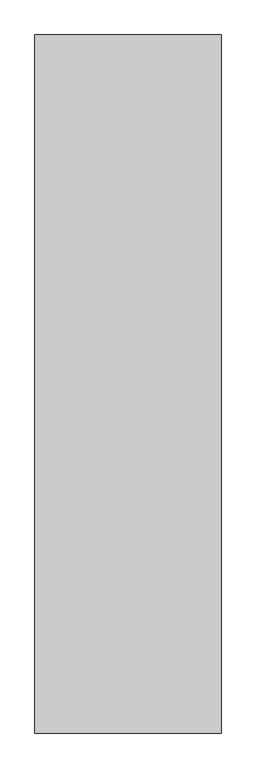
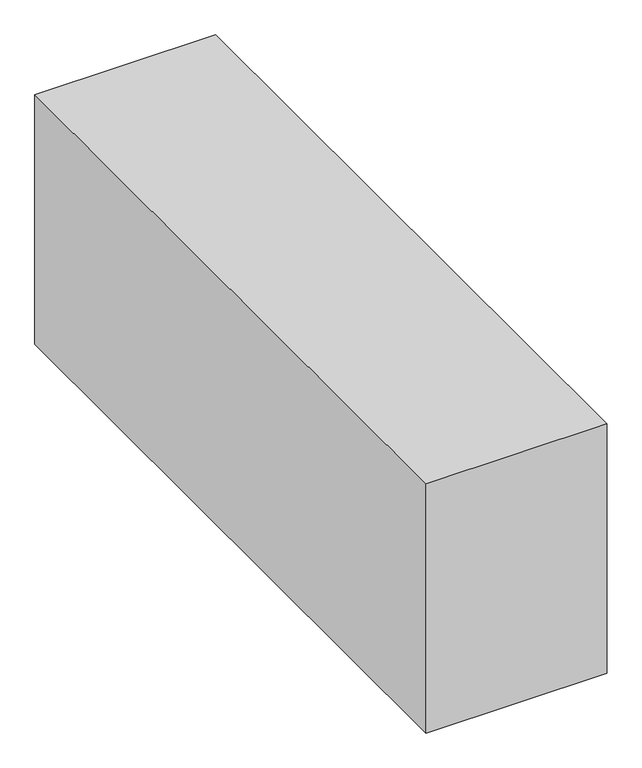
"""IFC4 building model written with IfcOpenShell, lengths in millimetres: proxy geometry, Space Planning Box_hec : Space Planning Box_hec."""

from ifc_helpers import new_model, si_unit, origin, origin_with_axes, place, context, project, spatial, polyline, outline, extrude, source, transform, mapped, element, save


def generic_models_3f6e5246(model_context):
    return source(origin(), model_context, "Body", "SweptSolid", [
        extrude(outline(polyline([(1200.0, 4500.0), (1200.0, -4500.0), (-1200.0, -4500.0), (-1200.0, 4500.0), (1200.0, 4500.0)])), origin_with_axes(), (0.0, 0.0, 1.0), 3500.0),
    ])


if __name__ == "__main__":
    model = new_model("IFC4")
    model_context = context("Model", 3, world=origin())
    ifc_project = project(units=[si_unit("LENGTHUNIT", "METRE", prefix="MILLI")], contexts=[model_context])
    site = spatial("IfcSite", under=ifc_project)
    building = spatial("IfcBuilding", under=site)
    placement = place(None, origin())
    generic_models_shape = generic_models_3f6e5246(model_context)
    element("IfcBuildingElementProxy", 1, Name="Space Planning Box_hec : Space Planning Box_hec", ObjectType="Space Planning Box_hec : Space Planning Box_hec", at=placement, inside=building, context=model_context, shape_type="MappedRepresentation", body=[
        mapped(generic_models_shape, transform((0.0, 0.0, 0.0), x_axis=(1.0, 0.0, 0.0), y_axis=(0.0, 1.0, 0.0), z_axis=(0.0, 0.0, 1.0))),
    ])
    save(model, "model.ifc")

# Revit data of these elements
# Type "Space Planning Box_hec : Space Planning Box_hec"
#   Type Comments = "..."
#   Room Name [instance default] = "?"
#   Interior Finish [instance default] = ""
#   Exterior Finish [instance default] = ""
#   Department [instance default] = ""
#   Assembly Code = "..."
#   ceiling height [instance default] = 0
#   Width [instance default] = 1524 mm
#   Program Area [instance default] = 0.00 m²
#   Length [instance default] = 1524 mm
#   Height [instance default] = 1524 mm
#   Area [instance default] = 2.32258 m²
#   Fill Color [instance default] = Cyan
#   Default Elevation = 0
# Element 1 (IfcBuildingElementProxy, "Space Planning Box_hec : Space Planning Box_hec")
#   Room Name = "Duct Shaft"
#   Exterior Finish = "RF1..N/A,,EW2..N/A..N/A"
#   Department = "PATHV3"
#   Width = 2400 mm
#   Program Area = 21.60 m²
#   Length = 9000 mm
#   Height = 3500 mm
#   Area = 21.60 m²
#   Fill Color = Lavender
#   Materials on its faces: "Lavender"
# Materials
#   "Cyan": class "Generic", colour RGB 0 255 255, transparency 0.2, Cost = 0
#   "Lavender": class "Generic", colour RGB 186 85 211, transparency 0.2, Cost = 0
